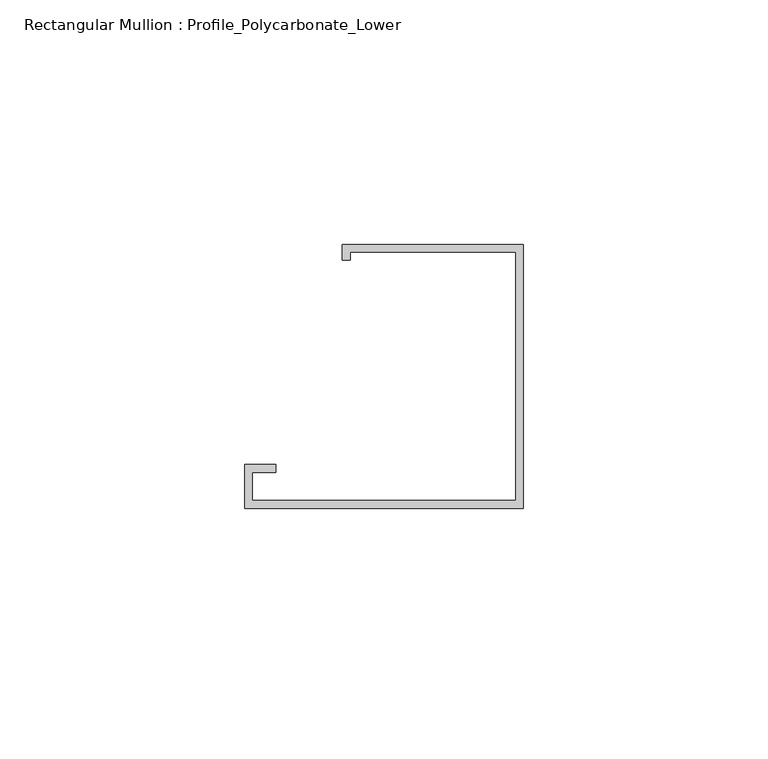
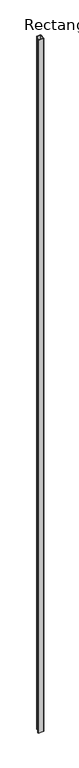
"""IFC4 building model written with IfcOpenShell, lengths in millimetres: member geometry, Rectangular Mullion : Profile_Polycarbonate_Lower."""

from ifc_helpers import new_model, si_unit, frame, origin, place, context, project, spatial, polyline, outline, extrude, source, transform, mapped, element, save


def rectangular_mullion_profile_polycarbonate_lower_07d50a76(model_context):
    return source(origin(), model_context, "Body", "SweptSolid", [
        extrude(outline(polyline([(0.0, -28.984575), (-56.9976, -28.984575), (-56.9976, -19.992975), (-50.6476, -19.992975), (-50.6476, -21.580475), (-55.4101, -21.580475), (-55.4101, -27.397075), (-1.5875, -27.397075), (-1.5875, 23.428325), (-35.3949, 23.428325), (-35.3949, 21.840825), (-36.9824, 21.840825), (-36.9824, 25.015825), (0.0, 25.015825), (0.0, -28.984575)])), frame((0.0, 0.0, -7162.9524), z_axis=(0.0, 0.0, 1.0), x_axis=(1.0, 0.0, 0.0)), (0.0, 0.0, 1.0), 7162.9524),
    ])


if __name__ == "__main__":
    model = new_model("IFC4")
    model_context = context("Model", 3, world=origin())
    ifc_project = project(units=[si_unit("LENGTHUNIT", "METRE", prefix="MILLI")], contexts=[model_context])
    site = spatial("IfcSite", under=ifc_project)
    building = spatial("IfcBuilding", under=site)
    placement = place(None, origin())
    rectangular_mullion_profile_polycarbonate_lower_shape = rectangular_mullion_profile_polycarbonate_lower_07d50a76(model_context)
    element("IfcMember", 1, ObjectType="Rectangular Mullion : Profile_Polycarbonate_Lower", at=placement, inside=building, context=model_context, shape_type="MappedRepresentation", body=[
        mapped(rectangular_mullion_profile_polycarbonate_lower_shape, transform((0.0, 0.0, 0.0), x_axis=(1.0, 0.0, 0.0), y_axis=(0.0, 1.0, 0.0), z_axis=(0.0, 0.0, 1.0))),
    ])
    save(model, "model.ifc")

# Revit data of these elements
# Type "Rectangular Mullion : Profile_Polycarbonate_Lower"
#   built-in parameter 1007322 = 0.177167 (stored number, unit not read)
#   built-in parameter 1007321 = 0 (stored number, unit not read)
#   built-in parameter 1007320 = 0.00520833 (stored number, unit not read)
